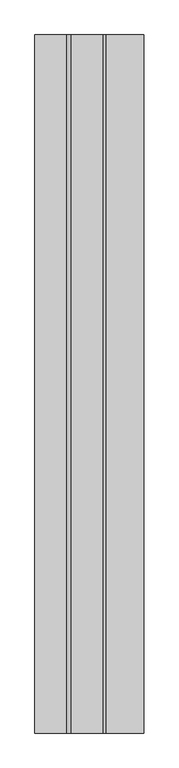
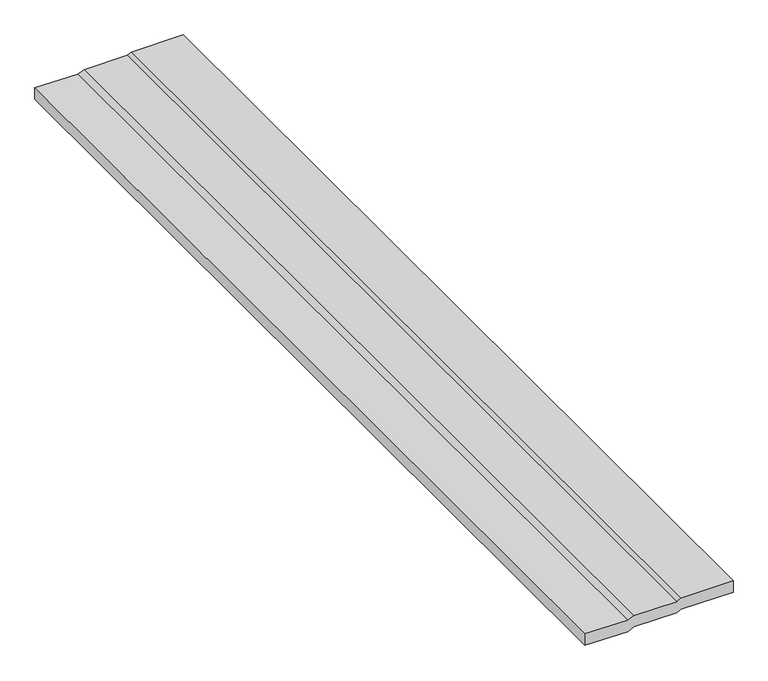
"""IFC4 building model written with IfcOpenShell, lengths in millimetres: proxy geometry, Gravel004 3869 : Gravel004 3869."""

from ifc_helpers import new_model, si_unit, frame, origin, place, context, project, spatial, polyline, outline, extrude, source, transform, mapped, element, save


def generic_models_468a0762(model_context):
    return source(origin(), model_context, "Body", "SweptSolid", [
        extrude(outline(polyline([(40274.2359464, -4497.235977), (40274.2359464, -4387.7364653), (40298.9742277, -4387.7364653), (40298.9742277, -4497.235977), (40294.6929777, -4505.9464262), (40294.6929777, -4596.5333403), (40288.9655157, -4609.3779796), (40290.6109464, -4699.8063764), (40265.8726651, -4699.8063764), (40264.2272344, -4609.3779796), (40269.9546964, -4596.5333403), (40269.9546964, -4505.9464262), (40274.2359464, -4497.235977)])), frame((0.0, -1052.6406573, 0.0), z_axis=(0.0, 1.0, 0.0), x_axis=(0.0, 0.0, 1.0)), (0.0, 0.0, 1.0), 2000.0),
    ])


if __name__ == "__main__":
    model = new_model("IFC4")
    model_context = context("Model", 3, world=origin())
    ifc_project = project(units=[si_unit("LENGTHUNIT", "METRE", prefix="MILLI")], contexts=[model_context])
    site = spatial("IfcSite", under=ifc_project)
    building = spatial("IfcBuilding", under=site)
    placement = place(None, origin())
    generic_models_shape = generic_models_468a0762(model_context)
    element("IfcBuildingElementProxy", 1, Name="Gravel004 3869 : Gravel004 3869", ObjectType="Gravel004 3869 : Gravel004 3869", at=placement, inside=building, context=model_context, shape_type="MappedRepresentation", body=[
        mapped(generic_models_shape, transform((0.0, 0.0, 0.0), x_axis=(1.0, 0.0, 0.0), y_axis=(0.0, 1.0, 0.0), z_axis=(0.0, 0.0, 1.0))),
    ])
    save(model, "model.ifc")

# Revit data of these elements
# Type "Gravel004 3869 : Gravel004 3869"
#   NameOverride = "Gravel004"
# Element 1 (IfcBuildingElementProxy, "Gravel004 3869 : Gravel004 3869")
#   Materials on its faces: "GRAVEL BALLAST"
# Materials
#   "GRAVEL BALLAST": class "Unassigned", colour RGB 128 128 128, transparency 0, Cost = 0
